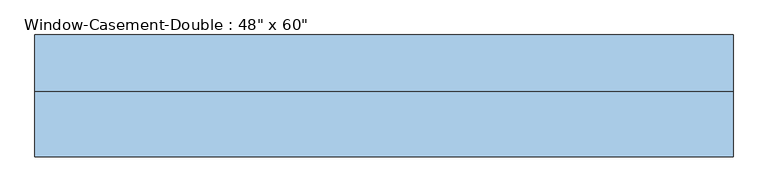
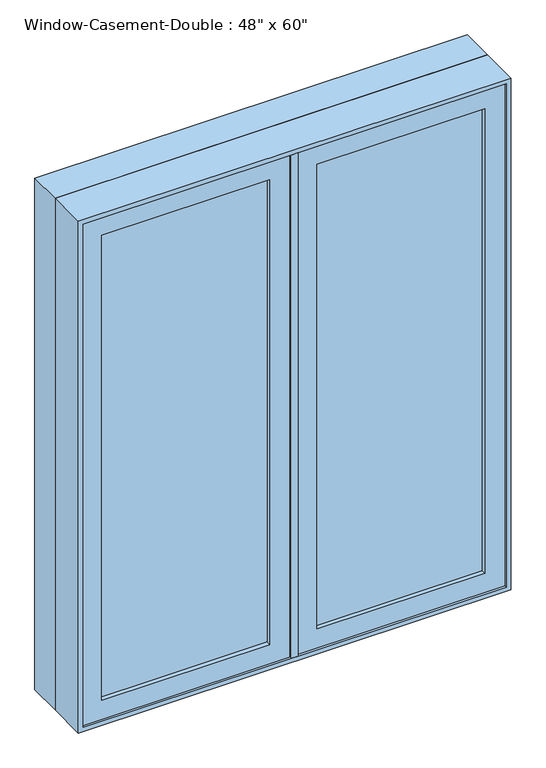
"""IFC4 building model written with IfcOpenShell, lengths in millimetres: window geometry."""

from ifc_helpers import new_model, si_unit, frame, origin, place, context, project, spatial, polyline, outline, extrude, faceted_brep, source, transform, mapped, element, save


def window_1e0f6214(model_context):
    return source(origin(), model_context, "Body", "SolidModel", [
        faceted_brep([(9.525, -115.8875, 2425.7), (9.525, -65.0875, 2425.7), (-9.525, -65.0875, 2425.7), (-9.525, -115.8875, 2425.7), (9.525, -115.8875, 927.1), (-9.525, -115.8875, 927.1), (-9.525, -65.0875, 927.1), (9.525, -65.0875, 927.1), (-9.525, -65.0875, 2406.65), (-9.525, -65.0875, 946.15), (-30.1625, -65.0875, 2406.65), (-30.1625, -65.0875, 946.15), (-30.1625, -1.5875, 2406.65), (-30.1625, -1.5875, 946.15), (30.1625, -1.5875, 2406.65), (30.1625, -1.5875, 946.15), (30.1625, -65.0875, 2406.65), (30.1625, -65.0875, 946.15), (9.525, -65.0875, 2406.65), (9.525, -65.0875, 946.15)], [[[0, 1, 2, 3]], [[4, 5, 6, 7]], [[3, 5, 4, 0]], [[2, 8, 9, 6, 5, 3]], [[8, 10, 11, 9]], [[10, 12, 13, 11]], [[12, 14, 15, 13]], [[14, 16, 17, 15]], [[16, 18, 19, 17]], [[0, 4, 7, 19, 18, 1]], [[8, 2, 1, 18]], [[19, 7, 6, 9]], [[9, 11, 13, 15, 17, 19]], [[18, 16, 14, 12, 10, 8]]]),
        extrude(outline(polyline([(-66.675, -96.8375), (-539.75, -96.8375), (-539.75, -90.4875), (-66.675, -90.4875), (-66.675, -96.8375)])), frame((0.0, 0.0, 984.25), z_axis=(0.0, 0.0, 1.0), x_axis=(1.0, 0.0, 0.0)), (0.0, 0.0, 1.0), 1384.3),
        extrude(outline(polyline([(-539.75, -77.7875), (-66.675, -77.7875), (-66.675, -84.1375), (-539.75, -84.1375), (-539.75, -77.7875)])), frame((0.0, 0.0, 984.25), z_axis=(0.0, 0.0, 1.0), x_axis=(1.0, 0.0, 0.0)), (0.0, 0.0, 1.0), 1384.3),
        extrude(outline(polyline([(539.75, -96.8375), (66.675, -96.8375), (66.675, -90.4875), (539.75, -90.4875), (539.75, -96.8375)])), frame((0.0, 0.0, 984.25), z_axis=(0.0, 0.0, 1.0), x_axis=(1.0, 0.0, 0.0)), (0.0, 0.0, 1.0), 1384.3),
        extrude(outline(polyline([(66.675, -77.7875), (539.75, -77.7875), (539.75, -84.1375), (66.675, -84.1375), (66.675, -77.7875)])), frame((0.0, 0.0, 984.25), z_axis=(0.0, 0.0, 1.0), x_axis=(1.0, 0.0, 0.0)), (0.0, 0.0, 1.0), 1384.3),
        extrude(outline(polyline([(2425.7, -9.525), (2425.7, -596.9), (927.1, -596.9), (927.1, -9.525), (2425.7, -9.525)]), holes=[polyline([(2368.55, -539.75), (2368.55, -66.675), (984.25, -66.675), (984.25, -539.75), (2368.55, -539.75)])]), frame((0.0, -109.5375, 0.0), z_axis=(0.0, 1.0, 0.0), x_axis=(0.0, 0.0, 1.0)), (0.0, 0.0, 1.0), 44.45),
        extrude(outline(polyline([(927.1, 9.525), (927.1, 596.9), (2425.7, 596.9), (2425.7, 9.525), (927.1, 9.525)]), holes=[polyline([(984.25, 539.75), (984.25, 66.675), (2368.55, 66.675), (2368.55, 539.75), (984.25, 539.75)])]), frame((0.0, -109.5375, 0.0), z_axis=(0.0, 1.0, 0.0), x_axis=(0.0, 0.0, 1.0)), (0.0, 0.0, 1.0), 44.45),
        extrude(outline(polyline([(2438.4, -609.6), (914.4, -609.6), (914.4, 609.6), (2438.4, 609.6), (2438.4, -609.6)]), holes=[polyline([(2419.35, 590.55), (933.45, 590.55), (933.45, -590.55), (2419.35, -590.55), (2419.35, 590.55)])]), frame((0.0, -1.5875, 0.0), z_axis=(0.0, 1.0, 0.0), x_axis=(0.0, 0.0, 1.0)), (0.0, 0.0, 1.0), 98.425),
        faceted_brep([(577.85, -65.0875, 2406.65), (-577.85, -65.0875, 2406.65), (-577.85, -1.5875, 2406.65), (577.85, -1.5875, 2406.65), (596.9, -115.8875, 2425.7), (-596.9, -115.8875, 2425.7), (-596.9, -65.0875, 2425.7), (596.9, -65.0875, 2425.7), (609.6, -1.5875, 2438.4), (-609.6, -1.5875, 2438.4), (-609.6, -115.8875, 2438.4), (609.6, -115.8875, 2438.4), (-577.85, -65.0875, 946.15), (-577.85, -1.5875, 946.15), (-596.9, -115.8875, 927.1), (-596.9, -65.0875, 927.1), (-609.6, -1.5875, 914.4), (-609.6, -115.8875, 914.4), (577.85, -65.0875, 946.15), (577.85, -1.5875, 946.15), (596.9, -115.8875, 927.1), (596.9, -65.0875, 927.1), (609.6, -1.5875, 914.4), (609.6, -115.8875, 914.4)], [[[0, 1, 2, 3]], [[4, 5, 6, 7]], [[8, 9, 10, 11]], [[1, 12, 13, 2]], [[5, 14, 15, 6]], [[9, 16, 17, 10]], [[12, 18, 19, 13]], [[14, 20, 21, 15]], [[16, 22, 23, 17]], [[9, 8, 22, 16], [3, 2, 13, 19]], [[18, 0, 3, 19]], [[7, 6, 15, 21], [1, 0, 18, 12]], [[20, 4, 7, 21]], [[22, 8, 11, 23]], [[11, 10, 17, 23], [5, 4, 20, 14]]]),
    ])


if __name__ == "__main__":
    model = new_model("IFC4")
    model_context = context("Model", 3, world=origin())
    ifc_project = project(units=[si_unit("LENGTHUNIT", "METRE", prefix="MILLI")], contexts=[model_context])
    site = spatial("IfcSite", under=ifc_project)
    building = spatial("IfcBuilding", under=site)
    placement = place(None, origin())
    window_shape = window_1e0f6214(model_context)
    element("IfcWindow", 1, ObjectType="Window-Casement-Double : 48\" x 60\"", at=placement, inside=building, context=model_context, shape_type="MappedRepresentation", body=[
        mapped(window_shape, transform((0.0, 0.0, 0.0), x_axis=(1.0, 0.0, 0.0), y_axis=(0.0, 1.0, 0.0), z_axis=(0.0, 0.0, 1.0))),
    ])
    save(model, "model.ifc")

# Revit data of these elements
# Project information
#   Project Issue Date = "Issue Date"
#   Project Status = "Project Status"
#   Client Name = "Owner"
#   Project Address = "Enter address here"
#   Project Name = "Project Name"
#   Project Number = "Project Number"
# Type "Window-Casement-Double : 48\" x 60\""
#   Type Mark = "61"
#   Fire Rating = "0.5h"
#   Assembly Code = "B2020100"
#   Analytic Construction = "Double glazing - domestic"
#   Frame Extension [instance default] = 0' - 0 1/4"
#   Window Inset [instance default] = 0' - 0"
#   Wall Thickness [instance default] = 0' - 6"
#   Interior Wall Closure [instance default] = 0' - 2 1/4"
#   Half Width = 2' - 0"
#   Visual Light Transmittance = 0.81
#   Thermal Resistance (R) = 1.8146 (h·ft²·°F)/BTU
#   Solar Heat Gain Coefficient = 0.76
#   Rough Width = 4' - 0 1/2"
#   Rough Height = 5' - 0 1/2"
#   Height = 5' - 0"
#   Heat Transfer Coefficient (U) = 0.5511 BTU/(h·ft²·°F)
#   Exterior Wall Closure [instance default] = 0' - 1 1/4"
#   Extension Jamb [instance default] = 0' - 2 1/4"
#   Default Sill Height = 3' - 0"
#   Width = 4' - 0"
#   Define Thermal Properties by = 0
#   Muntin Visibility = yes
#   Interior Trim Visibility [instance default] = yes
#   Exterior Trim Visibility [instance default] = yes
#   Extension Jamb Visibility [instance default] = yes
#   Interior Trim Material = Wood - Stained
#   Muntin Pattern = Muntin Pattern_2x2 : Muntin Pattern_2x2
#   Interior Trim = Trim-Window-Interior-Flat : Picture Frame
#   Interior Frame Material = Wood - Stained
#   Glass Panel Material = Glass
#   Exterior Trim Material = Clad - White
#   Exterior Trim = Trim-Window-Exterior-Flat : with Sill
#   Exterior Frame Material = Clad - White
#   Wall Closure = (empty or 0)
# Element 1 (IfcWindow, "Window-Casement-Double : 48\" x 60\"")
#   Wall Thickness = 0' - 7 5/8"
#   Extension Jamb = 0' - 3 7/8"
#   Materials on its faces: "Wood - Stained", "Glass", "Clad - White"
# Materials
#   "Wood - Stained": class "Wood", colour RGB 224 178 126, transparency 0, Cost = 0
#   "Glass": class "Glass", colour RGB 236 240 239, transparency 0.5, Description = "Soda Lime Glass", Cost = 0
#   "Clad - White": class "Wood", colour RGB 216 216 204, transparency 0, Cost = 0
